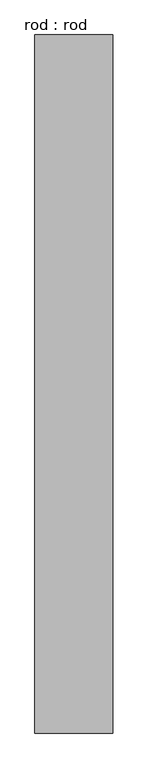
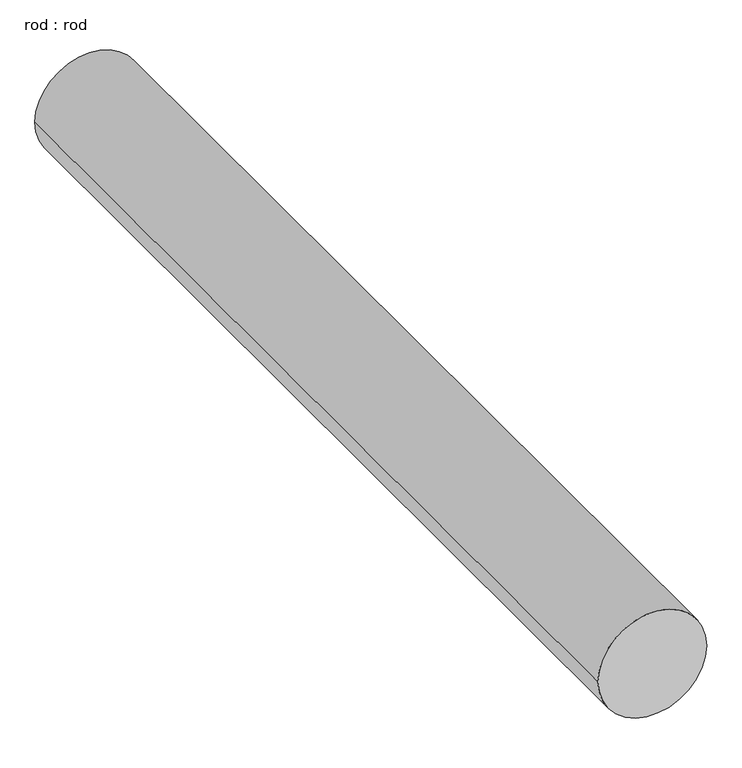
"""IFC4 building model written with IfcOpenShell, lengths in millimetres: proxy geometry, rod : rod."""

from ifc_helpers import new_model, si_unit, point, frame, frame_2d, origin, place, context, project, spatial, circle_curve, trimmed, segment, composite_curve, outline, extrude, source, transform, mapped, element, save


def rod_rod_629ab2bc(model_context):
    return source(origin(), model_context, "Body", "SweptSolid", [
        extrude(outline(composite_curve([segment(trimmed(circle_curve(frame_2d((0.0108462, 0.0)), 200.0), [point((0.0108462, 200.0))], [point((0.0108462, -200.0))], False, "CARTESIAN"), True, "CONTINUOUS"), segment(trimmed(circle_curve(frame_2d((0.0108462, 0.0)), 200.0), [point((0.0108462, -200.0))], [point((0.0108462, 200.0))], False, "CARTESIAN"), True, "CONTINUOUS")], self_intersect=False)), frame((0.0, 2298.0857582, 0.0), z_axis=(0.0, 1.0, 0.0), x_axis=(0.0, 0.0, 1.0)), (0.0, 0.0, 1.0), 3589.2857143),
    ])


if __name__ == "__main__":
    model = new_model("IFC4")
    model_context = context("Model", 3, world=origin())
    ifc_project = project(units=[si_unit("LENGTHUNIT", "METRE", prefix="MILLI")], contexts=[model_context])
    site = spatial("IfcSite", under=ifc_project)
    building = spatial("IfcBuilding", under=site)
    placement = place(None, origin())
    rod_rod_shape = rod_rod_629ab2bc(model_context)
    element("IfcBuildingElementProxy", 1, Name="rod : rod", ObjectType="rod : rod", at=placement, inside=building, context=model_context, shape_type="MappedRepresentation", body=[
        mapped(rod_rod_shape, transform((0.0, 0.0, 0.0), x_axis=(1.0, 0.0, 0.0), y_axis=(0.0, 1.0, 0.0), z_axis=(0.0, 0.0, 1.0))),
    ])
    save(model, "model.ifc")

# Revit data of these elements
# Type "rod : rod"
#   Default Elevation = 0
